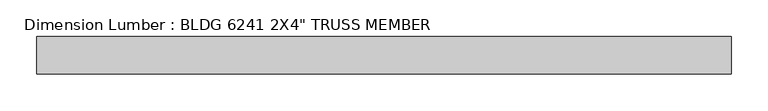
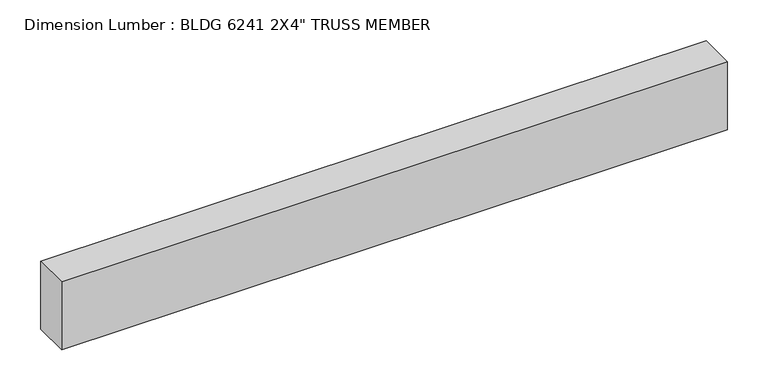
"""IFC4 building model written with IfcOpenShell, lengths in millimetres: beam geometry."""

from ifc_helpers import new_model, si_unit, frame, origin, place, context, project, spatial, polyline, outline, extrude, source, transform, mapped, element, save


def beam_f72471f4(model_context):
    return source(origin(), model_context, "Body", "SweptSolid", [
        extrude(outline(polyline([(482.6, 25.4), (482.6, -25.4), (-457.2, -25.4), (-457.2, 25.4), (482.6, 25.4)])), frame((0.0, 0.0, -50.8), z_axis=(0.0, 0.0, 1.0), x_axis=(1.0, 0.0, 0.0)), (0.0, 0.0, 1.0), 101.6),
    ])


if __name__ == "__main__":
    model = new_model("IFC4")
    model_context = context("Model", 3, world=origin())
    ifc_project = project(units=[si_unit("LENGTHUNIT", "METRE", prefix="MILLI")], contexts=[model_context])
    site = spatial("IfcSite", under=ifc_project)
    building = spatial("IfcBuilding", under=site)
    placement = place(None, origin())
    beam_shape = beam_f72471f4(model_context)
    element("IfcBeam", 1, ObjectType="Dimension Lumber : BLDG 6241 2X4\" TRUSS MEMBER", at=placement, inside=building, context=model_context, shape_type="MappedRepresentation", body=[
        mapped(beam_shape, transform((0.0, 0.0, 0.0), x_axis=(1.0, 0.0, 0.0), y_axis=(0.0, 1.0, 0.0), z_axis=(0.0, 0.0, 1.0))),
    ])
    save(model, "model.ifc")

# Revit data of these elements
# Type "Dimension Lumber : BLDG 6241 2X4\" TRUSS MEMBER"
#   Assembly Code = "B10"
#   A = 0.273472 SF
#   Length [instance default] = 5' - 0"
#   b = 0' - 2"
#   d = 0' - 4"
#   Structural Material [instance default] = Softwood, Lumber
# Element 1 (IfcBeam, "Dimension Lumber : BLDG 6241 2X4\" TRUSS MEMBER")
#   Materials on its faces: "Softwood, Lumber"
# Materials
#   "Softwood, Lumber": class "Wood", colour RGB 223 192 134, transparency 0, Description = "Pinus Echinata", Cost = 0
